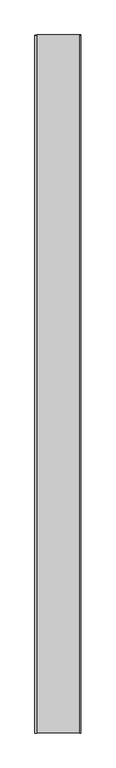
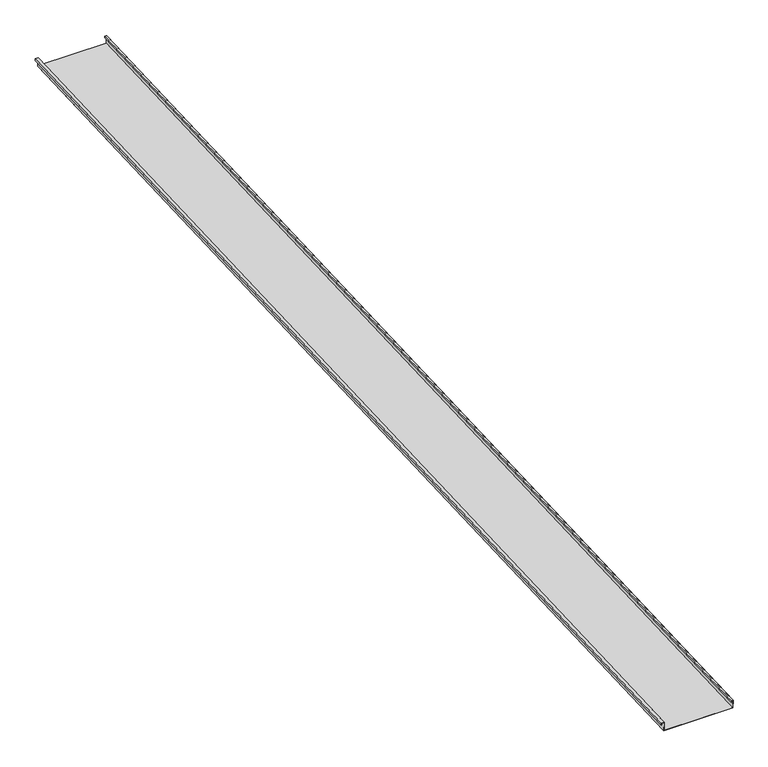
"""IFC4 building model written with IfcOpenShell, lengths in millimetres: proxy geometry, Generic Models 2:Generic Models 2:310765:Generic Models 2:310765 : Generic Models 2:Generic Models 2:310765:96 : Generic Models 2:Generic Models 2:310765:Generic Models 2:310765 : Generic Models 2:Generic Models 2:310765:300385."""

from ifc_helpers import new_model, si_unit, frame, origin, place, context, project, spatial, polyline, outline, extrude, source, transform, mapped, element, save


def generic_models_e5c510b4(model_context):
    return source(origin(), model_context, "Body", "SweptSolid", [
        extrude(outline(polyline([(1.5875, 0.0), (1.5875, 50.8), (407.9875, 50.8), (407.9875, 1.5875), (396.875, 1.5875), (396.875, 11.1125), (398.4625, 11.1125), (398.4625, 3.175), (406.4, 3.175), (406.4, 49.2125), (3.175, 49.2125), (3.175, -1.5874999), (-14.2875, -1.5874999), (-14.2875, 9.525), (-12.7, 9.525), (-12.7, 0.0), (1.5875, 0.0)])), frame((615596.1096406, -581354.4345603, 3902.6697972), z_axis=(0.0, 0.9991330730923568, 0.041630544712067834), x_axis=(1.0, 0.0, 0.0)), (0.0, 0.0, 1.0), 6400.8),
    ])


if __name__ == "__main__":
    model = new_model("IFC4")
    model_context = context("Model", 3, world=origin())
    ifc_project = project(units=[si_unit("LENGTHUNIT", "METRE", prefix="MILLI")], contexts=[model_context])
    site = spatial("IfcSite", under=ifc_project)
    building = spatial("IfcBuilding", under=site)
    placement = place(None, origin())
    generic_models_shape = generic_models_e5c510b4(model_context)
    element("IfcBuildingElementProxy", 1, Name="Generic Models 2:Generic Models 2:310765:Generic Models 2:310765 : Generic Models 2:Generic Models 2:310765:96 : Generic Models 2:Generic Models 2:310765:Generic Models 2:310765 : Generic Models 2:Generic Models 2:310765:300385", ObjectType="Generic Models 2:Generic Models 2:310765:Generic Models 2:310765 : Generic Models 2:Generic Models 2:310765:96 : Generic Models 2:Generic Models 2:310765:Generic Models 2:310765 : Generic Models 2:Generic Models 2:310765:300385", at=placement, inside=building, context=model_context, shape_type="MappedRepresentation", body=[
        mapped(generic_models_shape, transform((0.0, 0.0, 0.0), x_axis=(1.0, 0.0, 0.0), y_axis=(0.0, 1.0, 0.0), z_axis=(0.0, 0.0, 1.0))),
    ])
    save(model, "model.ifc")

# Revit data of these elements
# Type "Generic Models 2:Generic Models 2:310765:Generic Models 2:310765 : Generic Models 2:Generic Models 2:310765:96 : Generic Models 2:Generic Models 2:310765:Generic Models 2:310765 : Generic Models 2:Generic Models 2:310765:300385"
#   NameOverride = "Generic Models 2:Generic Models 2:310765:Generic Models 2:310765 : Generic Models 2:Generic Models 2:310765:300385"
#   ObjectTypeOverride = "Generic Models 2:310765 : Generic Models 2:Generic Models 2:310765"
#   Reference = "Generic Models 2"
#   Tag = "300385"
# Element 1 (IfcBuildingElementProxy, "Generic Models 2:Generic Models 2:310765:Generic Models 2:310765 : Generic Models 2:Generic Models 2:310765:96 : Generic Models 2:Generic Models 2:310765:Generic Models 2:310765 : Generic Models 2:Generic Models 2:310765:300385")
#   Materials on its faces: "THERMAL BROKEN ALUMINUM STOREFRONT FOR POLYCARBONATE"
# Materials
#   "THERMAL BROKEN ALUMINUM STOREFRONT FOR POLYCARBONATE": class "Unassigned", colour RGB 244 244 244, transparency 0, Keynote = "M07611300.01", Cost = 0
